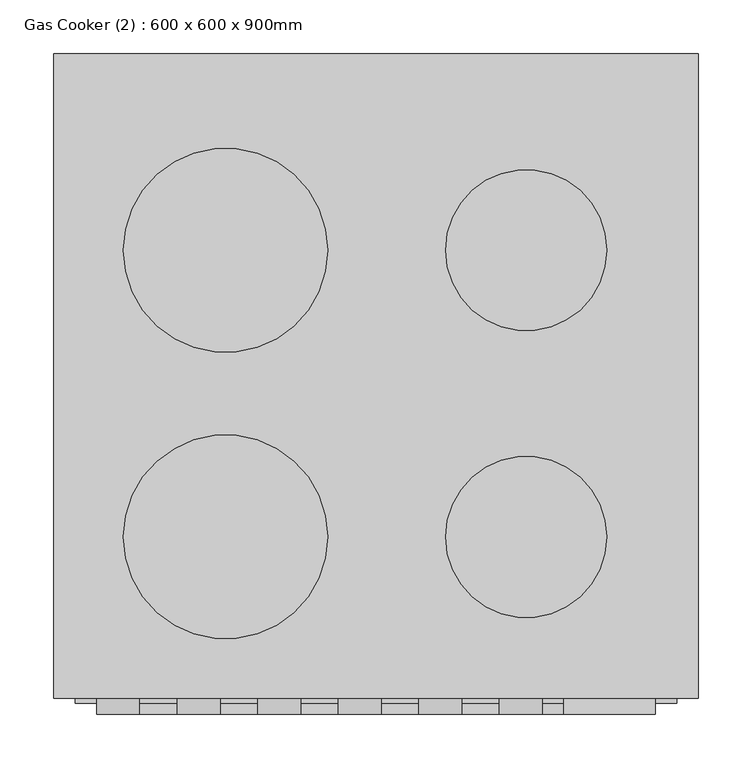
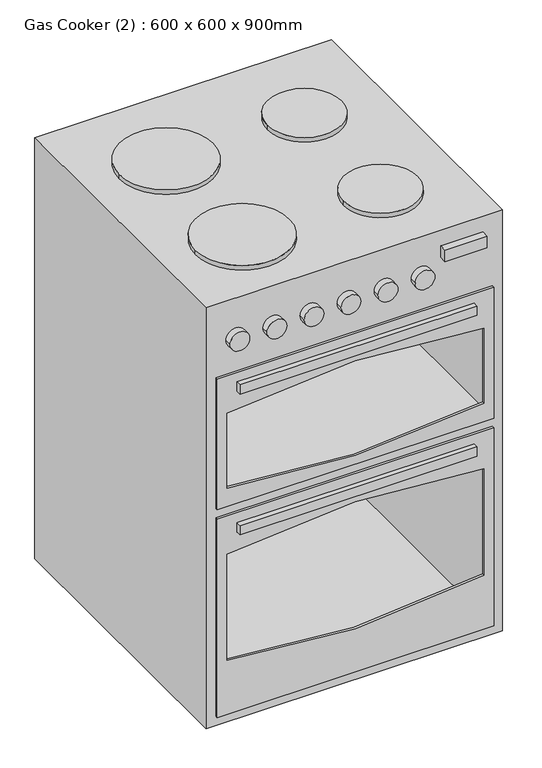
"""IFC4 building model written with IfcOpenShell, lengths in millimetres: proxy geometry, Gas Cooker (2) : 600 x 600 x 900mm."""

from ifc_helpers import new_model, si_unit, point, frame, frame_2d, origin, place, context, project, spatial, polyline, circle_curve, trimmed, segment, composite_curve, outline, extrude, faceted_brep, source, transform, mapped, element, save


def gas_cooker_2_600_x_600_x_900mm_b15ac652(model_context):
    return source(origin(), model_context, "Body", "SolidModel", [
        faceted_brep([(0.0, 10.0, 900.0), (0.0, 610.0, 900.0), (0.0, 610.0, 0.0), (0.0, 10.0, 0.0), (600.0, 10.0, 900.0), (600.0, 10.0, 0.0), (600.0, 610.0, 0.0), (600.0, 610.0, 900.0), (580.0, 10.0, 744.0), (580.0, 10.0, 464.0), (20.0, 10.0, 464.0), (20.0, 10.0, 744.0), (580.0, 10.0, 444.0), (580.0, 10.0, 20.0), (20.0, 10.0, 20.0), (20.0, 10.0, 444.0), (580.0, 577.0, 744.0), (20.0, 577.0, 744.0), (20.0, 577.0, 464.0), (580.0, 577.0, 464.0), (580.0, 577.0, 444.0), (20.0, 577.0, 444.0), (20.0, 577.0, 20.0), (580.0, 577.0, 20.0)], [[[0, 1, 2, 3]], [[4, 5, 6, 7]], [[1, 0, 4, 7]], [[2, 1, 7, 6]], [[3, 2, 6, 5]], [[0, 3, 5, 4], [8, 9, 10, 11], [12, 13, 14, 15]], [[16, 17, 18, 19]], [[20, 21, 22, 23]], [[16, 19, 9, 8]], [[19, 18, 10, 9]], [[18, 17, 11, 10]], [[17, 16, 8, 11]], [[20, 23, 13, 12]], [[23, 22, 14, 13]], [[22, 21, 15, 14]], [[21, 20, 12, 15]]]),
        extrude(outline(polyline([(540.0, -5.0), (59.8886957, -5.0), (59.8886957, 10.0), (540.0, 10.0), (540.0, -5.0)])), frame((0.0, 0.0, 704.0), z_axis=(0.0, 0.0, 1.0), x_axis=(1.0, 0.0, 0.0)), (0.0, 0.0, 1.0), 20.0),
        extrude(outline(polyline([(540.0, -5.0), (59.8886957, -5.0), (59.8886957, 10.0), (540.0, 10.0), (540.0, -5.0)])), frame((0.0, 0.0, 402.8798754), z_axis=(0.0, 0.0, 1.0), x_axis=(1.0, 0.0, 0.0)), (0.0, 0.0, 1.0), 20.0),
        extrude(outline(polyline([(560.0, -5.0), (475.0, -5.0), (475.0, 10.0), (560.0, 10.0), (560.0, -5.0)])), frame((0.0, 0.0, 841.7423922), z_axis=(0.0, 0.0, 1.0), x_axis=(1.0, 0.0, 0.0)), (0.0, 0.0, 1.0), 25.0),
        extrude(outline(composite_curve([segment(trimmed(circle_curve(frame_2d((816.7954925, 59.8886957)), 20.0), [point((816.7954925, 39.8886957))], [point((816.7954925, 79.8886957))], False, "CARTESIAN"), True, "CONTINUOUS"), segment(trimmed(circle_curve(frame_2d((816.7954925, 59.8886957)), 20.0), [point((816.7954925, 79.8886957))], [point((816.7954925, 39.8886957))], False, "CARTESIAN"), True, "CONTINUOUS")], self_intersect=False)), frame((0.0, -5.0, 0.0), z_axis=(0.0, 1.0, 0.0), x_axis=(0.0, 0.0, 1.0)), (0.0, 0.0, 1.0), 15.0),
        extrude(outline(composite_curve([segment(trimmed(circle_curve(frame_2d((816.7954925, 134.8886957)), 20.0), [point((816.7954925, 114.8886957))], [point((816.7954925, 154.8886957))], False, "CARTESIAN"), True, "CONTINUOUS"), segment(trimmed(circle_curve(frame_2d((816.7954925, 134.8886957)), 20.0), [point((816.7954925, 154.8886957))], [point((816.7954925, 114.8886957))], False, "CARTESIAN"), True, "CONTINUOUS")], self_intersect=False)), frame((0.0, -5.0, 0.0), z_axis=(0.0, 1.0, 0.0), x_axis=(0.0, 0.0, 1.0)), (0.0, 0.0, 1.0), 15.0),
        extrude(outline(composite_curve([segment(trimmed(circle_curve(frame_2d((816.7954925, 209.8886957)), 20.0), [point((816.7954925, 189.8886957))], [point((816.7954925, 229.8886957))], False, "CARTESIAN"), True, "CONTINUOUS"), segment(trimmed(circle_curve(frame_2d((816.7954925, 209.8886957)), 20.0), [point((816.7954925, 229.8886957))], [point((816.7954925, 189.8886957))], False, "CARTESIAN"), True, "CONTINUOUS")], self_intersect=False)), frame((0.0, -5.0, 0.0), z_axis=(0.0, 1.0, 0.0), x_axis=(0.0, 0.0, 1.0)), (0.0, 0.0, 1.0), 15.0),
        extrude(outline(composite_curve([segment(trimmed(circle_curve(frame_2d((816.7954925, 284.8886957)), 20.0), [point((816.7954925, 264.8886957))], [point((816.7954925, 304.8886957))], False, "CARTESIAN"), True, "CONTINUOUS"), segment(trimmed(circle_curve(frame_2d((816.7954925, 284.8886957)), 20.0), [point((816.7954925, 304.8886957))], [point((816.7954925, 264.8886957))], False, "CARTESIAN"), True, "CONTINUOUS")], self_intersect=False)), frame((0.0, -5.0, 0.0), z_axis=(0.0, 1.0, 0.0), x_axis=(0.0, 0.0, 1.0)), (0.0, 0.0, 1.0), 15.0),
        extrude(outline(composite_curve([segment(trimmed(circle_curve(frame_2d((816.7954925, 359.8886957)), 20.0), [point((816.7954925, 339.8886957))], [point((816.7954925, 379.8886957))], False, "CARTESIAN"), True, "CONTINUOUS"), segment(trimmed(circle_curve(frame_2d((816.7954925, 359.8886957)), 20.0), [point((816.7954925, 379.8886957))], [point((816.7954925, 339.8886957))], False, "CARTESIAN"), True, "CONTINUOUS")], self_intersect=False)), frame((0.0, -5.0, 0.0), z_axis=(0.0, 1.0, 0.0), x_axis=(0.0, 0.0, 1.0)), (0.0, 0.0, 1.0), 15.0),
        extrude(outline(composite_curve([segment(trimmed(circle_curve(frame_2d((816.7954925, 434.8886957)), 20.0), [point((816.7954925, 414.8886957))], [point((816.7954925, 454.8886957))], False, "CARTESIAN"), True, "CONTINUOUS"), segment(trimmed(circle_curve(frame_2d((816.7954925, 434.8886957)), 20.0), [point((816.7954925, 454.8886957))], [point((816.7954925, 414.8886957))], False, "CARTESIAN"), True, "CONTINUOUS")], self_intersect=False)), frame((0.0, -5.0, 0.0), z_axis=(0.0, 1.0, 0.0), x_axis=(0.0, 0.0, 1.0)), (0.0, 0.0, 1.0), 15.0),
        extrude(outline(polyline([(744.0, 580.0), (744.0, 20.0), (464.0, 20.0), (464.0, 580.0), (744.0, 580.0)]), holes=[composite_curve([segment(trimmed(circle_curve(frame_2d((-929.8168104, 300.0)), 1614.8845237), [point((664.0, 40.0))], [point((664.0, 560.0))], True, "CARTESIAN"), True, "CONTINUOUS"), segment(polyline([(664.0, 560.0), (503.6090566, 560.0)]), True, "CONTINUOUS"), segment(trimmed(circle_curve(frame_2d((2097.5428697, 300.0)), 1615.0000001), [point((503.6090566, 560.0))], [point((503.6090566, 40.0))], True, "CARTESIAN"), True, "CONTINUOUS"), segment(polyline([(503.6090566, 40.0), (664.0, 40.0)]), True, "CONTINUOUS")], self_intersect=False)]), frame((0.0, 5.0, 0.0), z_axis=(0.0, 1.0, 0.0), x_axis=(0.0, 0.0, 1.0)), (0.0, 0.0, 1.0), 5.0),
        extrude(outline(polyline([(444.0, 20.0), (20.0, 20.0), (20.0, 580.0), (444.0, 580.0), (444.0, 20.0)]), holes=[composite_curve([segment(trimmed(circle_curve(frame_2d((-1230.936935, 300.0)), 1614.8845237), [point((362.8798754, 40.0))], [point((362.8798754, 560.0))], True, "CARTESIAN"), True, "CONTINUOUS"), segment(polyline([(362.8798754, 560.0), (135.3289393, 560.0)]), True, "CONTINUOUS"), segment(trimmed(circle_curve(frame_2d((1579.9102153, 300.0)), 1467.7925818), [point((135.3289393, 560.0))], [point((135.3289393, 40.0))], True, "CARTESIAN"), True, "CONTINUOUS"), segment(polyline([(135.3289393, 40.0), (362.8798754, 40.0)]), True, "CONTINUOUS")], self_intersect=False)]), frame((0.0, 5.0, 0.0), z_axis=(0.0, 1.0, 0.0), x_axis=(0.0, 0.0, 1.0)), (0.0, 0.0, 1.0), 5.0),
        extrude(outline(composite_curve([segment(trimmed(circle_curve(frame_2d((160.0, 427.0)), 95.0), [point((65.0, 427.0))], [point((255.0, 427.0))], False, "CARTESIAN"), True, "CONTINUOUS"), segment(trimmed(circle_curve(frame_2d((160.0, 427.0)), 95.0), [point((255.0, 427.0))], [point((65.0, 427.0))], False, "CARTESIAN"), True, "CONTINUOUS")], self_intersect=False)), frame((0.0, 0.0, 900.0), z_axis=(0.0, 0.0, 1.0), x_axis=(1.0, 0.0, 0.0)), (0.0, 0.0, 1.0), 10.0),
        extrude(outline(composite_curve([segment(trimmed(circle_curve(frame_2d((440.0, 427.0)), 75.0), [point((365.0, 427.0))], [point((515.0, 427.0))], False, "CARTESIAN"), True, "CONTINUOUS"), segment(trimmed(circle_curve(frame_2d((440.0, 427.0)), 75.0), [point((515.0, 427.0))], [point((365.0, 427.0))], False, "CARTESIAN"), True, "CONTINUOUS")], self_intersect=False)), frame((0.0, 0.0, 900.0), z_axis=(0.0, 0.0, 1.0), x_axis=(1.0, 0.0, 0.0)), (0.0, 0.0, 1.0), 10.0),
        extrude(outline(composite_curve([segment(trimmed(circle_curve(frame_2d((440.0, 160.0)), 75.0), [point((365.0, 160.0))], [point((515.0, 160.0))], False, "CARTESIAN"), True, "CONTINUOUS"), segment(trimmed(circle_curve(frame_2d((440.0, 160.0)), 75.0), [point((515.0, 160.0))], [point((365.0, 160.0))], False, "CARTESIAN"), True, "CONTINUOUS")], self_intersect=False)), frame((0.0, 0.0, 900.0), z_axis=(0.0, 0.0, 1.0), x_axis=(1.0, 0.0, 0.0)), (0.0, 0.0, 1.0), 10.0),
        extrude(outline(composite_curve([segment(trimmed(circle_curve(frame_2d((160.0, 160.0)), 95.0), [point((65.0, 160.0))], [point((255.0, 160.0))], False, "CARTESIAN"), True, "CONTINUOUS"), segment(trimmed(circle_curve(frame_2d((160.0, 160.0)), 95.0), [point((255.0, 160.0))], [point((65.0, 160.0))], False, "CARTESIAN"), True, "CONTINUOUS")], self_intersect=False)), frame((0.0, 0.0, 900.0), z_axis=(0.0, 0.0, 1.0), x_axis=(1.0, 0.0, 0.0)), (0.0, 0.0, 1.0), 10.0),
    ])


if __name__ == "__main__":
    model = new_model("IFC4")
    model_context = context("Model", 3, world=origin())
    ifc_project = project(units=[si_unit("LENGTHUNIT", "METRE", prefix="MILLI")], contexts=[model_context])
    site = spatial("IfcSite", under=ifc_project)
    building = spatial("IfcBuilding", under=site)
    placement = place(None, origin())
    gas_cooker_2_600_x_600_x_900mm_shape = gas_cooker_2_600_x_600_x_900mm_b15ac652(model_context)
    element("IfcBuildingElementProxy", 1, Name="Gas Cooker (2) : 600 x 600 x 900mm", ObjectType="Gas Cooker (2) : 600 x 600 x 900mm", at=placement, inside=building, context=model_context, shape_type="MappedRepresentation", body=[
        mapped(gas_cooker_2_600_x_600_x_900mm_shape, transform((0.0, 0.0, 0.0), x_axis=(1.0, 0.0, 0.0), y_axis=(0.0, 1.0, 0.0), z_axis=(0.0, 0.0, 1.0))),
    ])
    save(model, "model.ifc")

# Revit data of these elements
# Type "Gas Cooker (2) : 600 x 600 x 900mm"
#   Keynote = "N"
#   Depth = 0.6 m
#   Height = 0.9 m
#   Width = 0.6 m
#   Cooker Material = Metal - Stainless Steel
#   Default Elevation = 0
# Element 1 (IfcBuildingElementProxy, "Gas Cooker (2) : 600 x 600 x 900mm")
#   Materials on its faces: "Metal - Paint Finish - Dark Gray, Matte", "Metal - Stainless Steel"
# Materials
#   "Metal - Stainless Steel": class "Metal", colour RGB 200 200 200, transparency 0
#   "Metal - Paint Finish - Dark Gray, Matte": class "Não atribuído", colour RGB 98 98 98, transparency 0
